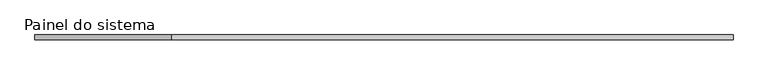
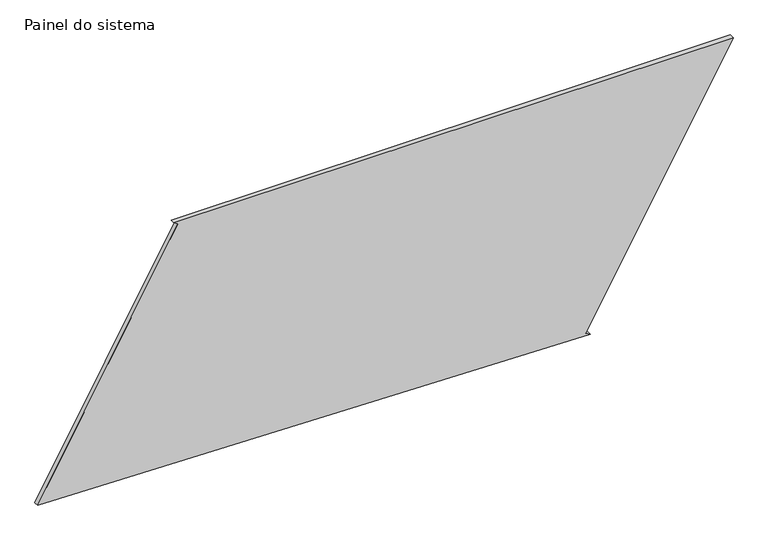
"""IFC4 building model written with IfcOpenShell, lengths in millimetres: plate geometry, Painel do sistema : Envidraçado."""

from ifc_helpers import new_model, si_unit, frame, origin, place, context, project, spatial, polyline, outline, extrude, source, transform, mapped, element, save


def painel_do_sistema_34a4bb8b(model_context):
    return source(origin(), model_context, "Body", "SweptSolid", [
        extrude(outline(polyline([(0.0, 1070.4735197), (12.2820845, 1048.6985249), (1376.730106, 1818.3090854), (1376.730106, -1106.6387274), (1364.4480214, -1084.8637326), (64.1175532, -1818.3090854), (0.0, 1070.4735197)])), frame((0.0, 24.5, 0.0), z_axis=(0.0, 1.0, 0.0), x_axis=(0.0, 0.0, 1.0)), (0.0, 0.0, 1.0), 25.0),
    ])


if __name__ == "__main__":
    model = new_model("IFC4")
    model_context = context("Model", 3, world=origin())
    ifc_project = project(units=[si_unit("LENGTHUNIT", "METRE", prefix="MILLI")], contexts=[model_context])
    site = spatial("IfcSite", under=ifc_project)
    building = spatial("IfcBuilding", under=site)
    placement = place(None, origin())
    painel_do_sistema_shape = painel_do_sistema_34a4bb8b(model_context)
    element("IfcPlate", 1, ObjectType="Painel do sistema : Envidraçado", at=placement, inside=building, context=model_context, shape_type="MappedRepresentation", body=[
        mapped(painel_do_sistema_shape, transform((0.0, 0.0, 0.0), x_axis=(1.0, 0.0, 0.0), y_axis=(0.0, 1.0, 0.0), z_axis=(0.0, 0.0, 1.0))),
    ])
    save(model, "model.ifc")

# Revit data of these elements
# Type "Painel do sistema : Envidraçado"
#   Construction Type Id = "GSP4R"
#   Analytic Construction = "Vidraça única Pilkington 1/8 pol"
#   Visual Light Transmittance = 0.9
#   Solar Heat Gain Coefficient = 0.86
#   Heat Transfer Coefficient (U) = 6.7069 W/(m²·K)
# Element 1 (IfcPlate, "Painel do sistema : Envidraçado")
#   Materials on its faces: "Vidro"
# Materials
#   "Vidro": class "Vidro", colour RGB 0 128 192, transparency 0.9, Description = "Vidro de sílica", Cost = 0
